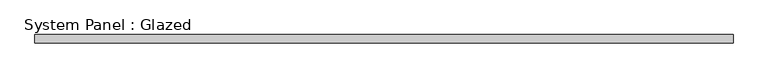
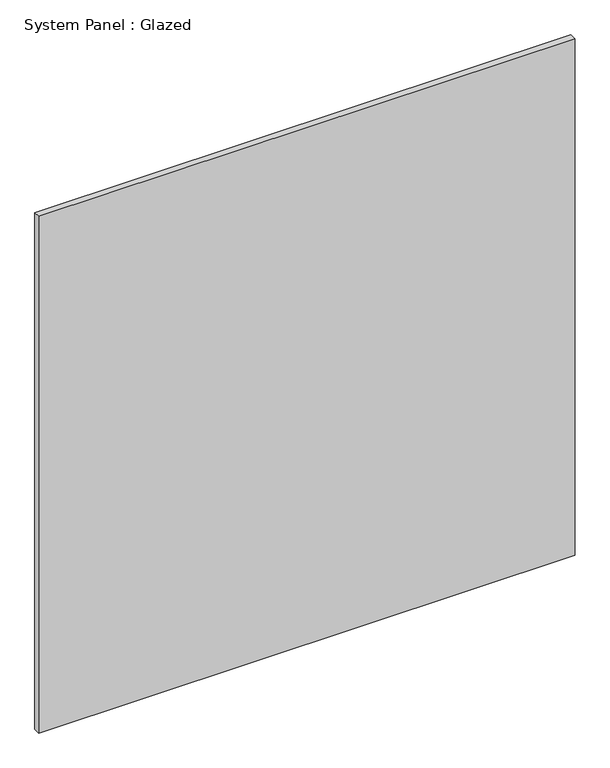
"""IFC4 building model written with IfcOpenShell, lengths in millimetres: plate geometry, System Panel : Glazed."""

from ifc_helpers import new_model, si_unit, origin, origin_with_axes, place, context, project, spatial, polyline, outline, extrude, source, transform, mapped, element, save


def system_panel_glazed_239482d2(model_context):
    return source(origin(), model_context, "Body", "SweptSolid", [
        extrude(outline(polyline([(1048.0594464, 24.5), (-1048.0594464, 24.5), (-1048.0594464, 49.5), (1048.0594464, 49.5), (1048.0594464, 24.5)])), origin_with_axes(), (0.0, 0.0, 1.0), 2134.9240943),
    ])


if __name__ == "__main__":
    model = new_model("IFC4")
    model_context = context("Model", 3, world=origin())
    ifc_project = project(units=[si_unit("LENGTHUNIT", "METRE", prefix="MILLI")], contexts=[model_context])
    site = spatial("IfcSite", under=ifc_project)
    building = spatial("IfcBuilding", under=site)
    placement = place(None, origin())
    system_panel_glazed_shape = system_panel_glazed_239482d2(model_context)
    element("IfcPlate", 1, ObjectType="System Panel : Glazed", at=placement, inside=building, context=model_context, shape_type="MappedRepresentation", body=[
        mapped(system_panel_glazed_shape, transform((0.0, 0.0, 0.0), x_axis=(1.0, 0.0, 0.0), y_axis=(0.0, 1.0, 0.0), z_axis=(0.0, 0.0, 1.0))),
    ])
    save(model, "model.ifc")

# Revit data of these elements
# Type "System Panel : Glazed"
#   Keynote = "H11"
#   Construction Type Id = "GSP4R"
#   Analytic Construction = "1/8 in Pilkington single glazing"
#   Visual Light Transmittance = 0.9
#   Solar Heat Gain Coefficient = 0.86
#   Heat Transfer Coefficient (U) = 6.7069 W/(m²·K)
#   Define Thermal Properties by = 1
# Element 1 (IfcPlate, "System Panel : Glazed")
#   Materials on its faces: "Glass"
# Materials
#   "Glass": class "Glass", colour RGB 0 128 192, transparency 0.9, Description = "Soda Lime Glass", Cost = 0
